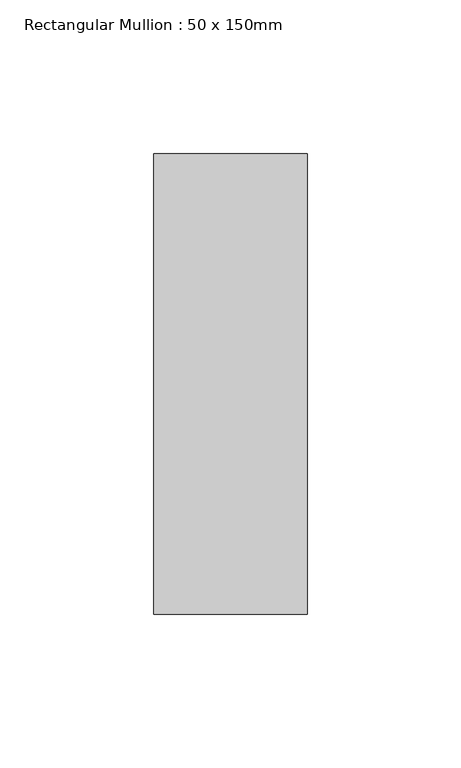
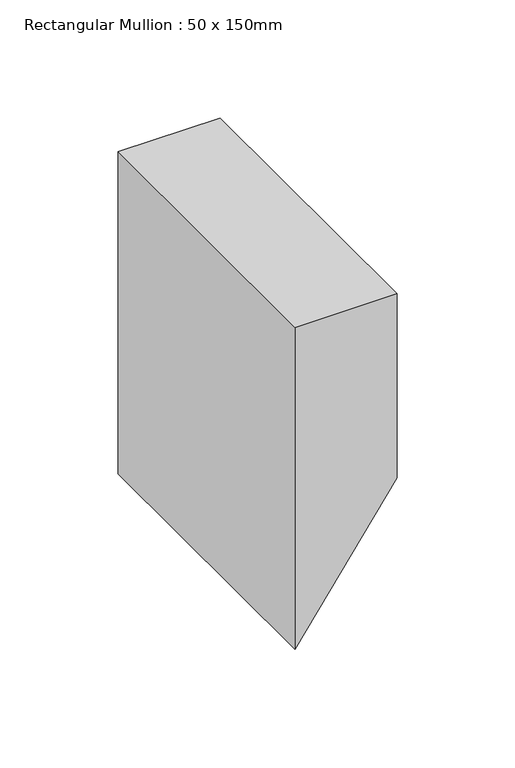
"""IFC4 building model written with IfcOpenShell, lengths in millimetres: member geometry, Rectangular Mullion : 50 x 150mm."""

import ifcopenshell
import ifcopenshell.guid

model = None  # the IFC model being written
_history = None  # IfcOwnerHistory: only IFC2X3 demands one
_inside = {}  # id of a spatial element -> (the spatial element, [elements in it])
_under = {}  # id of a project, library or spatial element -> (it, [spatial elements below it])
_declared = {}  # id of a project -> (the project, [libraries it declares])
_typed = {}  # id of a type object -> (the type object, [elements of that type])
_made_of = {}  # id of a material, layer set ... -> (it, [elements and type objects made of it])


def new_model(schema):
    """Start an empty IFC model of exactly this schema.

    Asked for "IFC4X3", IfcOpenShell would pick the latest addendum, in which some entities
    have other attributes; the version numbers below select the first issue.
    IFC2X3 requires an IfcOwnerHistory on every rooted entity: one is made here for all.
    """
    global model, _history
    if schema == "IFC4X3":
        model = ifcopenshell.file(schema_version=(4, 3, 0, 0))
    else:
        model = ifcopenshell.file(schema=schema)
    _inside.clear()
    _under.clear()
    _declared.clear()
    _typed.clear()
    _made_of.clear()
    _history = None
    if model.schema == "IFC2X3":
        org = make("IfcOrganization", Name="unknown")
        user = make(
            "IfcPersonAndOrganization",
            ThePerson=make("IfcPerson", FamilyName="unknown"),
            TheOrganization=org,
        )
        app = make(
            "IfcApplication",
            ApplicationDeveloper=org,
            Version="unknown",
            ApplicationFullName="unknown",
            ApplicationIdentifier="unknown",
        )
        _history = make(
            "IfcOwnerHistory",
            OwningUser=user,
            OwningApplication=app,
            ChangeAction="ADDED",
            CreationDate=0,
        )
    return model


def make(cls, **values):
    """One entity of the class cls with the attributes given. An attribute that is None is left unset."""
    return model.create_entity(
        cls, **{name: value for name, value in values.items() if value is not None}
    )


def rooted(cls, **values):
    """An entity with a GlobalId (a new one), such as an element, a storey or a relation."""
    return make(cls, GlobalId=ifcopenshell.guid.new(), OwnerHistory=_history, **values)


def si_unit(unit_type, name, prefix=None):
    """IfcSIUnit, for example si_unit("LENGTHUNIT", "METRE", prefix="MILLI")."""
    return make("IfcSIUnit", UnitType=unit_type, Prefix=prefix, Name=name)


def assignment(units):
    """IfcUnitAssignment: the units of a project."""
    return None if units is None else make("IfcUnitAssignment", Units=units)


def point(xyz):
    """IfcCartesianPoint."""
    return None if xyz is None else make("IfcCartesianPoint", Coordinates=xyz)


def direction(xyz):
    """IfcDirection."""
    return None if xyz is None else make("IfcDirection", DirectionRatios=xyz)


def frame(location, z_axis=None, x_axis=None):
    """IfcAxis2Placement3D, a coordinate frame: its origin and axes. An axis left out is left unset."""
    return make(
        "IfcAxis2Placement3D",
        Location=point(location),
        Axis=direction(z_axis),
        RefDirection=direction(x_axis),
    )


def origin():
    """The frame at (0, 0, 0) with its axes left unset."""
    return frame((0.0, 0.0, 0.0))


def place(relative_to, where):
    """IfcLocalPlacement: puts the frame where relative to a parent placement (None: the world)."""
    return make(
        "IfcLocalPlacement", PlacementRelTo=relative_to, RelativePlacement=where
    )


def context(
    kind, dimensions, precision=None, world=None, true_north=None, identifier=None
):
    """IfcGeometricRepresentationContext, for example the 3D "Model" context."""
    return make(
        "IfcGeometricRepresentationContext",
        ContextIdentifier=identifier,
        ContextType=kind,
        CoordinateSpaceDimension=dimensions,
        Precision=precision,
        WorldCoordinateSystem=world,
        TrueNorth=true_north,
    )


def project(units=None, contexts=None):
    """IfcProject with its units and contexts."""
    return rooted(
        "IfcProject",
        Name="project",
        RepresentationContexts=contexts,
        UnitsInContext=assignment(units),
    )


def spatial(cls, under=None, at=None, **own):
    """A site, building, storey or space (cls), placed at a placement, below another one or the project."""
    s = rooted(cls, ObjectPlacement=at, **own)
    if under is not None:
        _under.setdefault(under.id(), (under, []))[1].append(s)
    return s


def polyline(points):
    """IfcPolyline through the points."""
    return make("IfcPolyline", Points=[point(p) for p in points])


def outline(outer, holes=None, kind="AREA"):
    """IfcArbitraryClosedProfileDef: a profile drawn as a closed curve; with holes, ...WithVoids."""
    if holes is None:
        return make("IfcArbitraryClosedProfileDef", ProfileType=kind, OuterCurve=outer)
    return make(
        "IfcArbitraryProfileDefWithVoids",
        ProfileType=kind,
        OuterCurve=outer,
        InnerCurves=holes,
    )


def extrude(swept, where, along, depth):
    """IfcExtrudedAreaSolid: the profile swept, set in the frame where, extruded along a direction by depth."""
    return make(
        "IfcExtrudedAreaSolid",
        SweptArea=swept,
        Position=where,
        ExtrudedDirection=direction(along),
        Depth=depth,
    )


def shape(context_of_items, identifier, shape_type, items):
    """IfcShapeRepresentation: the items that make up one representation, for example the "Body"."""
    return make(
        "IfcShapeRepresentation",
        ContextOfItems=context_of_items,
        RepresentationIdentifier=identifier,
        RepresentationType=shape_type,
        Items=items,
    )


def source(mapping_origin, context_of_items, identifier, shape_type, items):
    """IfcRepresentationMap: a shape defined once, which mapped items show again and again."""
    return make(
        "IfcRepresentationMap",
        MappingOrigin=mapping_origin,
        MappedRepresentation=shape(context_of_items, identifier, shape_type, items),
    )


def transform(
    local_origin,
    x_axis=None,
    y_axis=None,
    z_axis=None,
    scale=None,
    scale2=None,
    scale3=None,
    uniform=True,
):
    """IfcCartesianTransformationOperator3D, or its non-uniform kind. x_axis, y_axis, z_axis: its Axis1, 2, 3."""
    if uniform:
        return make(
            "IfcCartesianTransformationOperator3D",
            Axis1=direction(x_axis),
            Axis2=direction(y_axis),
            LocalOrigin=point(local_origin),
            Scale=scale,
            Axis3=direction(z_axis),
        )
    return make(
        "IfcCartesianTransformationOperator3DnonUniform",
        Axis1=direction(x_axis),
        Axis2=direction(y_axis),
        LocalOrigin=point(local_origin),
        Scale=scale,
        Axis3=direction(z_axis),
        Scale2=scale2,
        Scale3=scale3,
    )


def mapped(mapping_source, mapping_target):
    """IfcMappedItem: shows the shape of a source again, moved by a transform."""
    return make(
        "IfcMappedItem", MappingSource=mapping_source, MappingTarget=mapping_target
    )


def made_of(thing, what):
    """Note that an element or type object is made of a material, layer set ...; save() writes the relation."""
    if what is not None:
        _made_of.setdefault(what.id(), (what, []))[1].append(thing)
    return thing


def element(
    cls,
    number,
    at=None,
    inside=None,
    cuts=None,
    type_object=None,
    material=None,
    context=None,
    identifier="Body",
    shape_type=None,
    held_by="IfcProductDefinitionShape",
    body=None,
    shapes=None,
    **own,
):
    """One element of the class cls, such as IfcWall. Its Tag is "e" and its number.

    at: its placement. inside: the storey or other place that contains it. cuts: it is an
    opening in that element (IfcRelVoidsElement). A single representation is given by context,
    identifier, shape_type and body (its items); several are given by shapes. held_by: the class
    of the entity that holds the representations. save() writes the other relations.
    """
    e = rooted(cls, Tag="e%d" % number, ObjectPlacement=at, **own)
    if body is not None:
        shapes = [shape(context, identifier, shape_type, body)]
    if shapes is not None:
        e.Representation = make(held_by, Representations=shapes)
    if inside is not None:
        _inside.setdefault(inside.id(), (inside, []))[1].append(e)
    if cuts is not None:
        rooted(
            "IfcRelVoidsElement", RelatingBuildingElement=cuts, RelatedOpeningElement=e
        )
    if type_object is not None:
        _typed.setdefault(type_object.id(), (type_object, []))[1].append(e)
    return made_of(e, material)


def aggregate(whole, parts):
    """IfcRelAggregates: a whole, such as a stair, and the parts it consists of."""
    return rooted("IfcRelAggregates", RelatingObject=whole, RelatedObjects=parts)


def save(model, path):
    """Write the relations noted so far, then the file.

    IfcRelAggregates (storeys below a building ...), IfcRelContainedInSpatialStructure (elements
    in a storey), IfcRelDefinesByType, IfcRelAssociatesMaterial and IfcRelDeclares: one each for
    every whole, place, type object, material and project.
    """
    for whole, parts in _under.values():
        aggregate(whole, parts)
    for where, things in _inside.values():
        rooted(
            "IfcRelContainedInSpatialStructure",
            RelatedElements=things,
            RelatingStructure=where,
        )
    for kind, things in _typed.values():
        rooted("IfcRelDefinesByType", RelatedObjects=things, RelatingType=kind)
    for what, things in _made_of.values():
        rooted("IfcRelAssociatesMaterial", RelatedObjects=things, RelatingMaterial=what)
    for by, libraries in _declared.values():
        rooted("IfcRelDeclares", RelatingContext=by, RelatedDefinitions=libraries)
    model.write(path)


def rectangular_mullion_50_x_150mm_544dbf8b(model_context):
    return source(origin(), model_context, "Body", "SweptSolid", [
        extrude(outline(polyline([(0.0, 25.0), (0.0, -25.0), (-166.6425563, -25.0), (-95.235156, 25.0), (0.0, 25.0)])), frame((0.0, -75.0, 0.0), z_axis=(0.0, 1.0, 0.0), x_axis=(0.0, 0.0, 1.0)), (0.0, 0.0, 1.0), 150.0),
    ])


if __name__ == "__main__":
    model = new_model("IFC4")
    model_context = context("Model", 3, world=origin())
    ifc_project = project(units=[si_unit("LENGTHUNIT", "METRE", prefix="MILLI")], contexts=[model_context])
    site = spatial("IfcSite", under=ifc_project)
    building = spatial("IfcBuilding", under=site)
    placement = place(None, origin())
    rectangular_mullion_50_x_150mm_shape = rectangular_mullion_50_x_150mm_544dbf8b(model_context)
    element("IfcMember", 1, ObjectType="Rectangular Mullion : 50 x 150mm", at=placement, inside=building, context=model_context, shape_type="MappedRepresentation", body=[
        mapped(rectangular_mullion_50_x_150mm_shape, transform((0.0, 0.0, 0.0), x_axis=(1.0, 0.0, 0.0), y_axis=(0.0, 1.0, 0.0), z_axis=(0.0, 0.0, 1.0))),
    ])
    save(model, "model.ifc")

# Revit data of these elements
# Type "Rectangular Mullion : 50 x 150mm"
#   built-in parameter 1007304 = 0.492126 (stored number, unit not read)
#   built-in parameter 1007301 = 0.082021 (stored number, unit not read)
#   built-in parameter 1007300 = 0.082021 (stored number, unit not read)
# Element 1 (IfcMember, "Rectangular Mullion : 50 x 150mm")
#   Materials on its faces: "Aluminium"
# Materials
#   "Aluminium": class "Metal", colour RGB 247 247 247, transparency 0, Description = "Aluminium 6061", Cost = 0
